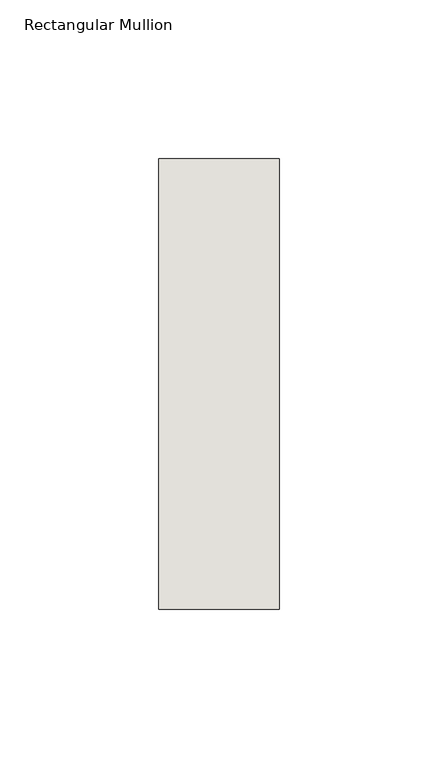
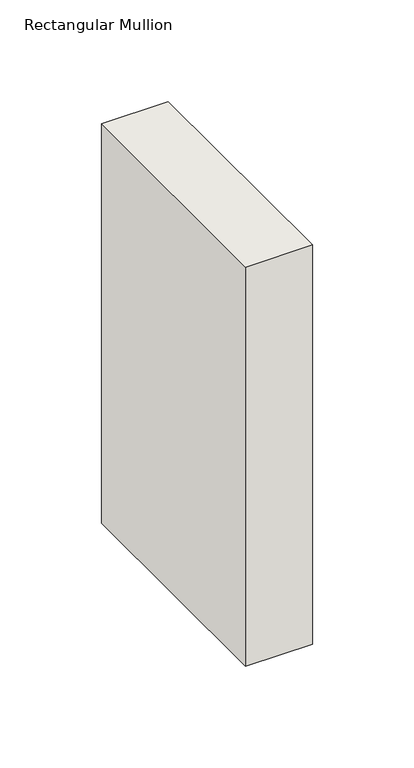
"""IFC4 building model written with IfcOpenShell, lengths in millimetres: wall geometry, Rectangular Mullion : NLRS_21_CWM_hsb-regel 38x142_gen_rsf."""

from ifc_helpers import new_model, si_unit, frame, origin, place, context, project, spatial, polyline, outline, extrude, source, transform, mapped, element, save


def rectangular_mullion_e6972d68(model_context):
    return source(origin(), model_context, "Body", "SweptSolid", [
        extrude(outline(polyline([(0.0, -71.0), (-38.0, -71.0), (-38.0, 71.0), (0.0, 71.0), (0.0, -71.0)])), frame((0.0, 0.0, -239.8441061), z_axis=(0.0, 0.0, 1.0), x_axis=(1.0, 0.0, 0.0)), (0.0, 0.0, 1.0), 239.8441061),
    ])


if __name__ == "__main__":
    model = new_model("IFC4")
    model_context = context("Model", 3, world=origin())
    ifc_project = project(units=[si_unit("LENGTHUNIT", "METRE", prefix="MILLI")], contexts=[model_context])
    site = spatial("IfcSite", under=ifc_project)
    building = spatial("IfcBuilding", under=site)
    placement = place(None, origin())
    rectangular_mullion_shape = rectangular_mullion_e6972d68(model_context)
    element("IfcWall", 1, ObjectType="Rectangular Mullion : NLRS_21_CWM_hsb-regel 38x142_gen_rsf", at=placement, inside=building, context=model_context, shape_type="MappedRepresentation", body=[
        mapped(rectangular_mullion_shape, transform((0.0, 0.0, 0.0), x_axis=(1.0, 0.0, 0.0), y_axis=(0.0, 1.0, 0.0), z_axis=(0.0, 0.0, 1.0))),
    ])
    save(model, "model.ifc")

# Revit data of these elements
# Type "Rectangular Mullion : NLRS_21_CWM_hsb-regel 38x142_gen_rsf"
#   Type IfcGUID = "07M7mRoiH1CR8m_RSKIwpF"
#   Assembly Code = "21.10"
#   IfcExportAs = "IfcWall"
#   built-in parameter 1007322 = 0.465879 (stored number, unit not read)
#   built-in parameter 1007321 = 0.062336 (stored number, unit not read)
#   built-in parameter 1007320 = 0.062336 (stored number, unit not read)
# Element 1 (IfcWall, "Rectangular Mullion : NLRS_21_CWM_hsb-regel 38x142_gen_rsf")
#   Materials on its faces: "NLRS_i2_hout naaldhout vuren_gen_rsf"
# Materials
#   "NLRS_i2_hout naaldhout vuren_gen_rsf": class "I - Hout", colour RGB 234 199 147, transparency 0, Keynote = "i2", Manufacturer = "Revit Standards Foundation", URL = "www.revitstandards.org", Description = "hout vuren", Cost = 0
